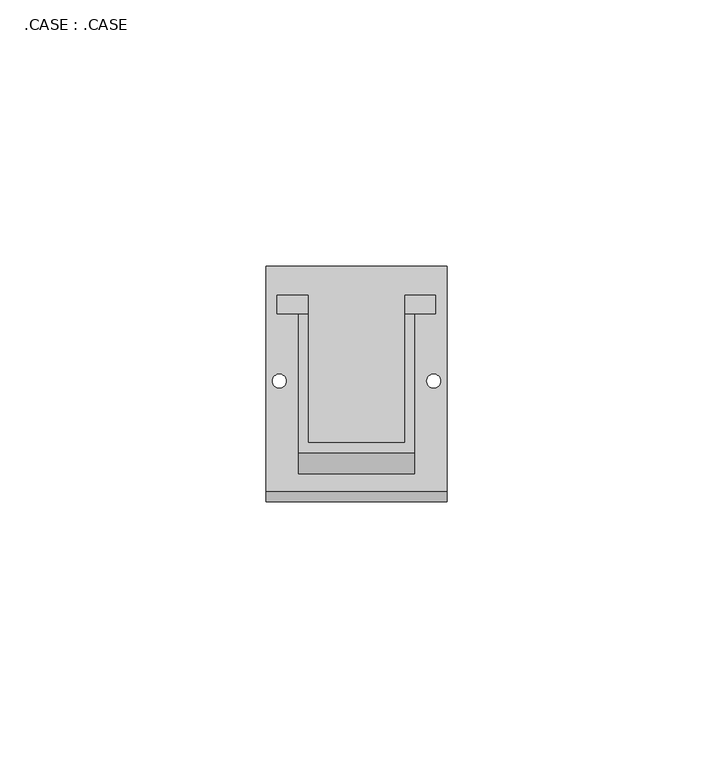
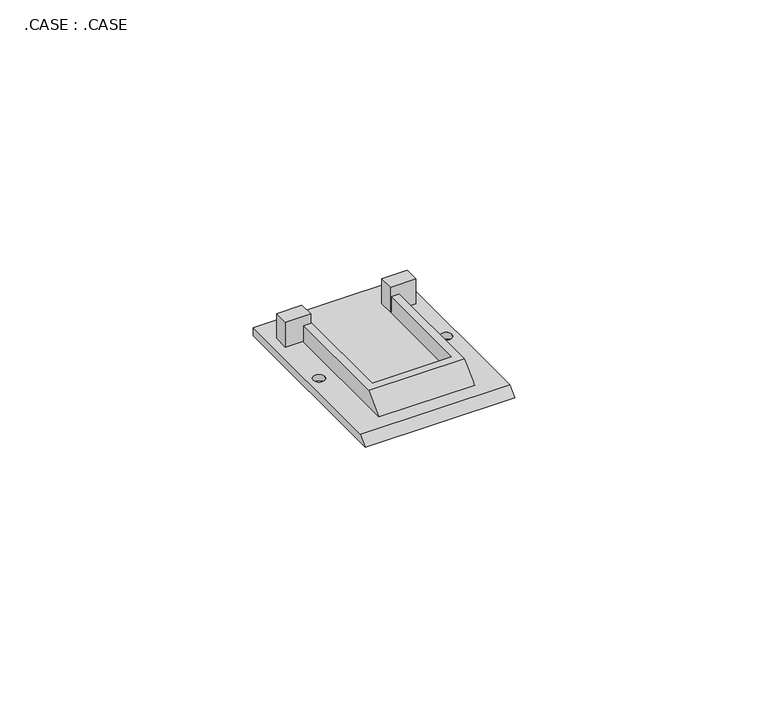
"""IFC4 building model written with IfcOpenShell, lengths in millimetres: proxy geometry, .CASE : .CASE."""

import ifcopenshell
import ifcopenshell.guid

model = None  # the IFC model being written
_history = None  # IfcOwnerHistory: only IFC2X3 demands one
_inside = {}  # id of a spatial element -> (the spatial element, [elements in it])
_under = {}  # id of a project, library or spatial element -> (it, [spatial elements below it])
_declared = {}  # id of a project -> (the project, [libraries it declares])
_typed = {}  # id of a type object -> (the type object, [elements of that type])
_made_of = {}  # id of a material, layer set ... -> (it, [elements and type objects made of it])


def new_model(schema):
    """Start an empty IFC model of exactly this schema.

    Asked for "IFC4X3", IfcOpenShell would pick the latest addendum, in which some entities
    have other attributes; the version numbers below select the first issue.
    IFC2X3 requires an IfcOwnerHistory on every rooted entity: one is made here for all.
    """
    global model, _history
    if schema == "IFC4X3":
        model = ifcopenshell.file(schema_version=(4, 3, 0, 0))
    else:
        model = ifcopenshell.file(schema=schema)
    _inside.clear()
    _under.clear()
    _declared.clear()
    _typed.clear()
    _made_of.clear()
    _history = None
    if model.schema == "IFC2X3":
        org = make("IfcOrganization", Name="unknown")
        user = make(
            "IfcPersonAndOrganization",
            ThePerson=make("IfcPerson", FamilyName="unknown"),
            TheOrganization=org,
        )
        app = make(
            "IfcApplication",
            ApplicationDeveloper=org,
            Version="unknown",
            ApplicationFullName="unknown",
            ApplicationIdentifier="unknown",
        )
        _history = make(
            "IfcOwnerHistory",
            OwningUser=user,
            OwningApplication=app,
            ChangeAction="ADDED",
            CreationDate=0,
        )
    return model


def make(cls, **values):
    """One entity of the class cls with the attributes given. An attribute that is None is left unset."""
    return model.create_entity(
        cls, **{name: value for name, value in values.items() if value is not None}
    )


def rooted(cls, **values):
    """An entity with a GlobalId (a new one), such as an element, a storey or a relation."""
    return make(cls, GlobalId=ifcopenshell.guid.new(), OwnerHistory=_history, **values)


def si_unit(unit_type, name, prefix=None):
    """IfcSIUnit, for example si_unit("LENGTHUNIT", "METRE", prefix="MILLI")."""
    return make("IfcSIUnit", UnitType=unit_type, Prefix=prefix, Name=name)


def assignment(units):
    """IfcUnitAssignment: the units of a project."""
    return None if units is None else make("IfcUnitAssignment", Units=units)


def point(xyz):
    """IfcCartesianPoint."""
    return None if xyz is None else make("IfcCartesianPoint", Coordinates=xyz)


def direction(xyz):
    """IfcDirection."""
    return None if xyz is None else make("IfcDirection", DirectionRatios=xyz)


def frame(location, z_axis=None, x_axis=None):
    """IfcAxis2Placement3D, a coordinate frame: its origin and axes. An axis left out is left unset."""
    return make(
        "IfcAxis2Placement3D",
        Location=point(location),
        Axis=direction(z_axis),
        RefDirection=direction(x_axis),
    )


def origin():
    """The frame at (0, 0, 0) with its axes left unset."""
    return frame((0.0, 0.0, 0.0))


def place(relative_to, where):
    """IfcLocalPlacement: puts the frame where relative to a parent placement (None: the world)."""
    return make(
        "IfcLocalPlacement", PlacementRelTo=relative_to, RelativePlacement=where
    )


def context(
    kind, dimensions, precision=None, world=None, true_north=None, identifier=None
):
    """IfcGeometricRepresentationContext, for example the 3D "Model" context."""
    return make(
        "IfcGeometricRepresentationContext",
        ContextIdentifier=identifier,
        ContextType=kind,
        CoordinateSpaceDimension=dimensions,
        Precision=precision,
        WorldCoordinateSystem=world,
        TrueNorth=true_north,
    )


def project(units=None, contexts=None):
    """IfcProject with its units and contexts."""
    return rooted(
        "IfcProject",
        Name="project",
        RepresentationContexts=contexts,
        UnitsInContext=assignment(units),
    )


def spatial(cls, under=None, at=None, **own):
    """A site, building, storey or space (cls), placed at a placement, below another one or the project."""
    s = rooted(cls, ObjectPlacement=at, **own)
    if under is not None:
        _under.setdefault(under.id(), (under, []))[1].append(s)
    return s


def polyline(points):
    """IfcPolyline through the points."""
    return make("IfcPolyline", Points=[point(p) for p in points])


def circle_curve(where, radius):
    """IfcCircle in the frame where."""
    return make("IfcCircle", Position=where, Radius=radius)


def outline(outer, holes=None, kind="AREA"):
    """IfcArbitraryClosedProfileDef: a profile drawn as a closed curve; with holes, ...WithVoids."""
    if holes is None:
        return make("IfcArbitraryClosedProfileDef", ProfileType=kind, OuterCurve=outer)
    return make(
        "IfcArbitraryProfileDefWithVoids",
        ProfileType=kind,
        OuterCurve=outer,
        InnerCurves=holes,
    )


def extrude(swept, where, along, depth):
    """IfcExtrudedAreaSolid: the profile swept, set in the frame where, extruded along a direction by depth."""
    return make(
        "IfcExtrudedAreaSolid",
        SweptArea=swept,
        Position=where,
        ExtrudedDirection=direction(along),
        Depth=depth,
    )


def shape(context_of_items, identifier, shape_type, items):
    """IfcShapeRepresentation: the items that make up one representation, for example the "Body"."""
    return make(
        "IfcShapeRepresentation",
        ContextOfItems=context_of_items,
        RepresentationIdentifier=identifier,
        RepresentationType=shape_type,
        Items=items,
    )


def source(mapping_origin, context_of_items, identifier, shape_type, items):
    """IfcRepresentationMap: a shape defined once, which mapped items show again and again."""
    return make(
        "IfcRepresentationMap",
        MappingOrigin=mapping_origin,
        MappedRepresentation=shape(context_of_items, identifier, shape_type, items),
    )


def transform(
    local_origin,
    x_axis=None,
    y_axis=None,
    z_axis=None,
    scale=None,
    scale2=None,
    scale3=None,
    uniform=True,
):
    """IfcCartesianTransformationOperator3D, or its non-uniform kind. x_axis, y_axis, z_axis: its Axis1, 2, 3."""
    if uniform:
        return make(
            "IfcCartesianTransformationOperator3D",
            Axis1=direction(x_axis),
            Axis2=direction(y_axis),
            LocalOrigin=point(local_origin),
            Scale=scale,
            Axis3=direction(z_axis),
        )
    return make(
        "IfcCartesianTransformationOperator3DnonUniform",
        Axis1=direction(x_axis),
        Axis2=direction(y_axis),
        LocalOrigin=point(local_origin),
        Scale=scale,
        Axis3=direction(z_axis),
        Scale2=scale2,
        Scale3=scale3,
    )


def mapped(mapping_source, mapping_target):
    """IfcMappedItem: shows the shape of a source again, moved by a transform."""
    return make(
        "IfcMappedItem", MappingSource=mapping_source, MappingTarget=mapping_target
    )


def made_of(thing, what):
    """Note that an element or type object is made of a material, layer set ...; save() writes the relation."""
    if what is not None:
        _made_of.setdefault(what.id(), (what, []))[1].append(thing)
    return thing


def element(
    cls,
    number,
    at=None,
    inside=None,
    cuts=None,
    type_object=None,
    material=None,
    context=None,
    identifier="Body",
    shape_type=None,
    held_by="IfcProductDefinitionShape",
    body=None,
    shapes=None,
    **own,
):
    """One element of the class cls, such as IfcWall. Its Tag is "e" and its number.

    at: its placement. inside: the storey or other place that contains it. cuts: it is an
    opening in that element (IfcRelVoidsElement). A single representation is given by context,
    identifier, shape_type and body (its items); several are given by shapes. held_by: the class
    of the entity that holds the representations. save() writes the other relations.
    """
    e = rooted(cls, Tag="e%d" % number, ObjectPlacement=at, **own)
    if body is not None:
        shapes = [shape(context, identifier, shape_type, body)]
    if shapes is not None:
        e.Representation = make(held_by, Representations=shapes)
    if inside is not None:
        _inside.setdefault(inside.id(), (inside, []))[1].append(e)
    if cuts is not None:
        rooted(
            "IfcRelVoidsElement", RelatingBuildingElement=cuts, RelatedOpeningElement=e
        )
    if type_object is not None:
        _typed.setdefault(type_object.id(), (type_object, []))[1].append(e)
    return made_of(e, material)


def aggregate(whole, parts):
    """IfcRelAggregates: a whole, such as a stair, and the parts it consists of."""
    return rooted("IfcRelAggregates", RelatingObject=whole, RelatedObjects=parts)


def save(model, path):
    """Write the relations noted so far, then the file.

    IfcRelAggregates (storeys below a building ...), IfcRelContainedInSpatialStructure (elements
    in a storey), IfcRelDefinesByType, IfcRelAssociatesMaterial and IfcRelDeclares: one each for
    every whole, place, type object, material and project.
    """
    for whole, parts in _under.values():
        aggregate(whole, parts)
    for where, things in _inside.values():
        rooted(
            "IfcRelContainedInSpatialStructure",
            RelatedElements=things,
            RelatingStructure=where,
        )
    for kind, things in _typed.values():
        rooted("IfcRelDefinesByType", RelatedObjects=things, RelatingType=kind)
    for what, things in _made_of.values():
        rooted("IfcRelAssociatesMaterial", RelatedObjects=things, RelatingMaterial=what)
    for by, libraries in _declared.values():
        rooted("IfcRelDeclares", RelatingContext=by, RelatedDefinitions=libraries)
    model.write(path)


def plane_surface(at):
    """IfcPlane: the flat surface through the origin of the frame at, square to its z axis."""
    return make("IfcPlane", Position=at)


def revolved_surface(curve, axis_point, axis_direction):
    """IfcSurfaceOfRevolution: the curve turned about the line through axis_point along axis_direction."""
    return make(
        "IfcSurfaceOfRevolution",
        SweptCurve=make("IfcArbitraryOpenProfileDef", ProfileType="CURVE", Curve=curve),
        AxisPosition=make("IfcAxis1Placement", Location=point(axis_point), Axis=direction(axis_direction)),
    )


def advanced_brep(points, edges, surfaces, faces):
    """IfcAdvancedBrep: a solid bounded by faces that lie on surfaces and meet in shared edges.

    An edge is (start, end): straight between two places in points (the first is 0);
    or (start, end, curve); or (start, end, curve, False) where it runs against its curve.
    A face is (place in surfaces, loops), or (place, loops, False) where it looks against
    its surface's normal. A loop lists edges by number (the first is 1), with a minus sign
    where the edge is run from its end to its start. The first loop is the outer one.
    """
    corners = [point(p) for p in points]
    vertices = [make("IfcVertexPoint", VertexGeometry=c) for c in corners]
    made = []
    for start, end, *more in edges:
        made.append(
            make(
                "IfcEdgeCurve",
                EdgeStart=vertices[start],
                EdgeEnd=vertices[end],
                EdgeGeometry=more[0] if more else make("IfcPolyline", Points=[corners[start], corners[end]]),
                SameSense=more[1] if len(more) > 1 else True,
            )
        )
    hull = []
    for where, loops, *sense in faces:
        bounds = []
        for j, loop in enumerate(loops):
            ring = [make("IfcOrientedEdge", EdgeElement=made[abs(k) - 1], Orientation=k > 0) for k in loop]
            bounds.append(
                make(
                    "IfcFaceOuterBound" if j == 0 else "IfcFaceBound",
                    Bound=make("IfcEdgeLoop", EdgeList=ring),
                    Orientation=True,
                )
            )
        hull.append(make("IfcAdvancedFace", Bounds=bounds, FaceSurface=surfaces[where], SameSense=sense[0] if sense else True))
    return make("IfcAdvancedBrep", Outer=make("IfcClosedShell", CfsFaces=hull))


def case_case_ec59ddf9(model_context):
    return source(origin(), model_context, "Body", "SolidModel", [
        extrude(outline(polyline([(1461.1150176, 13229.1739696), (1466.9150176, 13229.1739696), (1466.9150176, 13225.7186096), (1461.1150176, 13225.7186096), (1461.1150176, 13229.1739696)])), frame((0.0, 0.0, 2.0), z_axis=(0.0, 0.0, 1.0), x_axis=(1.0, 0.0, 0.0)), (0.0, 0.0, 1.0), 6.0),
        extrude(outline(polyline([(1442.9350176, 13229.1739696), (1442.9350176, 13225.7186096), (1437.1350176, 13225.7186096), (1437.1350176, 13229.1739696), (1442.9350176, 13229.1739696)])), frame((0.0, 0.0, 2.0), z_axis=(0.0, 0.0, 1.0), x_axis=(1.0, 0.0, 0.0)), (0.0, 0.0, 1.0), 6.0),
        advanced_brep(
        [(1469.0250176, 13192.4212784, 2.0), (1469.0250176, 13234.6739696, 2.0), (1435.0250176, 13234.6739696, 2.0), (1435.0250176, 13192.4212784, 2.0), (1441.1350176, 13195.6739696, 2.0), (1441.1350176, 13225.7186096, 2.0), (1442.9350176, 13225.7186096, 2.0), (1442.9350176, 13201.4739696, 2.0), (1461.1150176, 13201.4739696, 2.0), (1461.1150176, 13225.7186096, 2.0), (1462.9150176, 13225.7186096, 2.0), (1462.9150176, 13195.6739696, 2.0), (1467.8250176, 13213.1041412, 2.0), (1465.2250176, 13213.1041412, 2.0), (1438.8250176, 13213.1041412, 2.0), (1436.2250176, 13213.1041412, 2.0), (1435.0250176, 13234.6739696, 0.0), (1469.0250176, 13234.6739696, 0.0), (1469.0250176, 13190.4212784, 0.0), (1435.0250176, 13190.4212784, 0.0), (1464.5250176, 13213.1041412, 0.0), (1468.5250176, 13213.1041412, 0.0), (1435.5250176, 13213.1041412, 0.0), (1439.5250176, 13213.1041412, 0.0), (1441.1350176, 13225.7186096, 6.0), (1441.1350176, 13199.6739696, 6.0), (1462.9150176, 13199.6739696, 6.0), (1462.9150176, 13225.7186096, 6.0), (1461.1150176, 13225.7186096, 6.0), (1461.1150176, 13201.4739696, 6.0), (1442.9350176, 13201.4739696, 6.0), (1442.9350176, 13225.7186096, 6.0)],
        [
            (0, 1),
            (1, 2),
            (2, 3),
            (3, 0),
            (4, 5),
            (5, 6),
            (6, 7),
            (7, 8),
            (8, 9),
            (9, 10),
            (10, 11),
            (11, 4),
            (12, 13, circle_curve(frame((1466.5250176, 13213.1041412, 2.0), z_axis=(0.0, 0.0, -1.0), x_axis=(-1.0, 0.0, 0.0)), 1.3)),
            (13, 12, circle_curve(frame((1466.5250176, 13213.1041412, 2.0), z_axis=(0.0, 0.0, -1.0), x_axis=(1.0, 0.0, 0.0)), 1.3)),
            (14, 15, circle_curve(frame((1437.5250176, 13213.1041412, 2.0), z_axis=(0.0, 0.0, -1.0), x_axis=(-1.0, 0.0, 0.0)), 1.3)),
            (15, 14, circle_curve(frame((1437.5250176, 13213.1041412, 2.0), z_axis=(0.0, 0.0, -1.0), x_axis=(1.0, 0.0, 0.0)), 1.3)),
            (16, 17),
            (17, 18),
            (18, 19),
            (19, 16),
            (20, 21, circle_curve(frame((1466.5250176, 13213.1041412, 0.0), z_axis=(0.0, 0.0, 1.0), x_axis=(-1.0, 0.0, 0.0)), 2.0)),
            (21, 20, circle_curve(frame((1466.5250176, 13213.1041412, 0.0), z_axis=(0.0, 0.0, 1.0), x_axis=(1.0, 0.0, 0.0)), 2.0)),
            (22, 23, circle_curve(frame((1437.5250176, 13213.1041412, 0.0), z_axis=(0.0, 0.0, 1.0), x_axis=(-1.0, 0.0, 0.0)), 2.0)),
            (23, 22, circle_curve(frame((1437.5250176, 13213.1041412, 0.0), z_axis=(0.0, 0.0, 1.0), x_axis=(1.0, 0.0, 0.0)), 2.0)),
            (0, 18),
            (17, 1),
            (16, 2),
            (19, 3),
            (24, 25),
            (25, 26),
            (26, 27),
            (27, 28),
            (28, 29),
            (29, 30),
            (30, 31),
            (31, 24),
            (24, 5),
            (4, 25),
            (26, 11),
            (10, 27),
            (9, 28),
            (8, 29),
            (7, 30),
            (6, 31),
            (20, 13),
            (12, 21),
            (22, 15),
            (14, 23),
        ],
        [
            plane_surface(frame((1467.7850176, 13192.4212784, 2.0), z_axis=(0.0, 0.0, 1.0), x_axis=(1.0, 0.0, 0.0))),
            plane_surface(frame((1467.7850176, 13192.4212784, 0.0), z_axis=(0.0, 0.0, -1.0), x_axis=(-1.0, 0.0, 0.0))),
            plane_surface(frame((1469.0250176, 13192.4212784, 2.0), z_axis=(1.0, 0.0, 0.0), x_axis=(0.0, 0.0, -1.0))),
            plane_surface(frame((1469.0250176, 13234.6739696, 2.0), z_axis=(0.0, 1.0, 0.0), x_axis=(0.0, 0.0, -1.0))),
            plane_surface(frame((1435.0250176, 13234.6739696, 2.0), z_axis=(-1.0, 0.0, 0.0), x_axis=(0.0, 0.0, -1.0))),
            plane_surface(frame((1441.1350176, 13234.6739696, 6.0), z_axis=(0.0, 0.0, 1.0), x_axis=(0.0, -1.0, 0.0))),
            plane_surface(frame((1441.1350176, 13225.7186096, 6.0), z_axis=(-1.0, 0.0, 0.0), x_axis=(0.0, 0.0, -1.0))),
            plane_surface(frame((1462.9150176, 13199.6739696, 6.0), z_axis=(1.0, 0.0, 0.0), x_axis=(0.0, 0.0, -1.0))),
            plane_surface(frame((1462.9150176, 13225.7186096, 6.0), z_axis=(0.0, 1.0, 0.0), x_axis=(0.0, 0.0, -1.0))),
            plane_surface(frame((1461.1150176, 13225.7186096, 6.0), z_axis=(-1.0, 0.0, 0.0), x_axis=(0.0, 0.0, -1.0))),
            plane_surface(frame((1461.1150176, 13201.4739696, 6.0), z_axis=(0.0, 1.0, 0.0), x_axis=(0.0, 0.0, -1.0))),
            plane_surface(frame((1442.9350176, 13201.4739696, 6.0), z_axis=(1.0, 0.0, 0.0), x_axis=(0.0, 0.0, -1.0))),
            plane_surface(frame((1442.9350176, 13225.7186096, 6.0), z_axis=(0.0, 1.0, 0.0), x_axis=(0.0, 0.0, -1.0))),
            plane_surface(frame((1441.1350176, 13195.6739696, 2.0), z_axis=(0.0, -0.7071067811865885, 0.7071067811865066), x_axis=(1.0, 0.0, 0.0))),
            plane_surface(frame((1435.0250176, 13190.4212784, 0.0), z_axis=(0.0, -0.707106781186628, 0.7071067811864672), x_axis=(1.0, 0.0, 0.0))),
            revolved_surface(polyline([(1464.5250176, 13213.1041412, 0.0), (1465.2250176017499, 13213.1041412, 2.0)]), (1466.5250176, 13213.1041412, 5.7142857), (0.0, 0.0, -1.0)),
            revolved_surface(polyline([(1435.5250176, 13213.1041412, 0.0), (1436.2250176017499, 13213.1041412, 2.0)]), (1437.5250176, 13213.1041412, 5.7142857), (0.0, 0.0, -1.0)),
        ],
        [
            (0, [[1, 2, 3, 4], [5, 6, 7, 8, 9, 10, 11, 12], [13, 14], [15, 16]]),
            (1, [[17, 18, 19, 20], [21, 22], [23, 24]]),
            (2, [[-1, 25, -18, 26]]),
            (3, [[-2, -26, -17, 27]]),
            (4, [[-3, -27, -20, 28]]),
            (5, [[29, 30, 31, 32, 33, 34, 35, 36]]),
            (6, [[-29, 37, -5, 38]]),
            (7, [[-31, 39, -11, 40]]),
            (8, [[-32, -40, -10, 41]]),
            (9, [[-33, -41, -9, 42]]),
            (10, [[-34, -42, -8, 43]]),
            (11, [[-35, -43, -7, 44]]),
            (12, [[-36, -44, -6, -37]]),
            (13, [[-38, -12, -39, -30]]),
            (14, [[-28, -19, -25, -4]]),
            (15, [[45, -13, 46, -21]]),
            (15, [[-45, -22, -46, -14]]),
            (16, [[47, -15, 48, -23]]),
            (16, [[-47, -24, -48, -16]]),
        ],
    ),
    ])


if __name__ == "__main__":
    model = new_model("IFC4")
    model_context = context("Model", 3, world=origin())
    ifc_project = project(units=[si_unit("LENGTHUNIT", "METRE", prefix="MILLI")], contexts=[model_context])
    site = spatial("IfcSite", under=ifc_project)
    building = spatial("IfcBuilding", under=site)
    placement = place(None, origin())
    case_case_shape = case_case_ec59ddf9(model_context)
    element("IfcBuildingElementProxy", 1, Name=".CASE : .CASE", ObjectType=".CASE : .CASE", at=placement, inside=building, context=model_context, shape_type="MappedRepresentation", body=[
        mapped(case_case_shape, transform((0.0, 0.0, 0.0), x_axis=(1.0, 0.0, 0.0), y_axis=(0.0, 1.0, 0.0), z_axis=(0.0, 0.0, 1.0))),
    ])
    save(model, "model.ifc")

# Revit data of these elements
# Element 1 (IfcBuildingElementProxy, ".CASE : .CASE")
#   Materials on its faces: "Areia"
# Materials
#   "Areia": class "Genérico", colour RGB 191 183 178, transparency 0, Description = "Areia", Cost = 0
